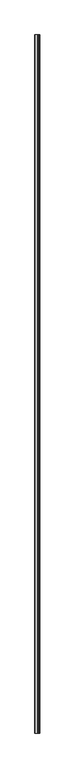
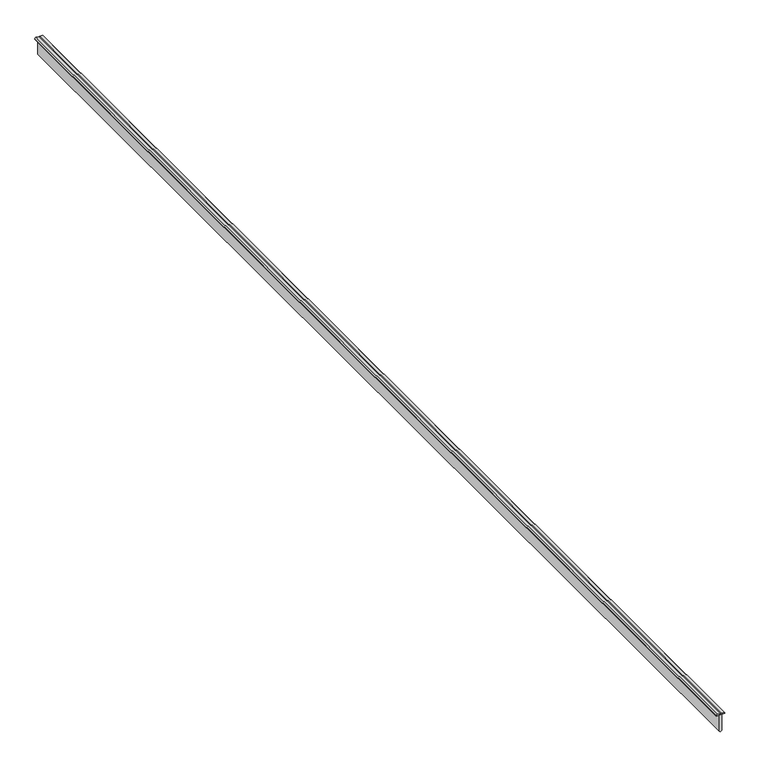
"""IFC4 building model written with IfcOpenShell, lengths in millimetres: proxy geometry, FASTENER 1:FASTENER 11861:297350 : FASTENER 1:FASTENER 11861:297350."""

from ifc_helpers import new_model, si_unit, frame, origin, place, context, project, spatial, polyline, outline, extrude, source, transform, mapped, element, save


def generic_models_a558a684(model_context):
    return source(origin(), model_context, "Body", "SweptSolid", [
        extrude(outline(polyline([(42582.1288635, 10750.5257946), (42580.5349921, 10749.2870925), (42579.6987049, 10749.2762959), (42579.6987049, 10763.5726012), (42580.508527, 10763.5726012), (42582.1023984, 10762.3338991), (42582.1023984, 10757.4548172), (42580.1167322, 10757.0482169), (42580.1167322, 10755.801112), (42581.7222633, 10755.801112), (42582.1288635, 10750.5257946)])), frame((0.0, -774.5581163, 0.0), z_axis=(0.0, 1.0, 0.0), x_axis=(0.0, 0.0, 1.0)), (0.0, 0.0, 1.0), 1999.85),
        extrude(outline(polyline([(42549.1244121, 10755.9768301), (42551.3049701, 10758.526734), (42579.6987049, 10758.526734), (42579.6987049, 10754.3198155), (42550.7399648, 10754.3198155), (42549.1244121, 10755.9768301)])), frame((0.0, -774.5581163, 0.0), z_axis=(0.0, 1.0, 0.0), x_axis=(0.0, 0.0, 1.0)), (0.0, 0.0, 1.0), 1999.85),
    ])


if __name__ == "__main__":
    model = new_model("IFC4")
    model_context = context("Model", 3, world=origin())
    ifc_project = project(units=[si_unit("LENGTHUNIT", "METRE", prefix="MILLI")], contexts=[model_context])
    site = spatial("IfcSite", under=ifc_project)
    building = spatial("IfcBuilding", under=site)
    placement = place(None, origin())
    generic_models_shape = generic_models_a558a684(model_context)
    element("IfcBuildingElementProxy", 1, Name="FASTENER 1:FASTENER 11861:297350 : FASTENER 1:FASTENER 11861:297350", ObjectType="FASTENER 1:FASTENER 11861:297350 : FASTENER 1:FASTENER 11861:297350", at=placement, inside=building, context=model_context, shape_type="MappedRepresentation", body=[
        mapped(generic_models_shape, transform((0.0, 0.0, 0.0), x_axis=(1.0, 0.0, 0.0), y_axis=(0.0, 1.0, 0.0), z_axis=(0.0, 0.0, 1.0))),
    ])
    save(model, "model.ifc")

# Revit data of these elements
# Type "FASTENER 1:FASTENER 11861:297350 : FASTENER 1:FASTENER 11861:297350"
#   NameOverride = "FASTENER 1:FASTENER 11861:297350"
#   ObjectTypeOverride = "FASTENER 1:FASTENER 11861"
#   Reference = "FASTENER 11861"
#   Category = "Generic Models"
#   Tag = "297350"
# Element 1 (IfcBuildingElementProxy, "FASTENER 1:FASTENER 11861:297350 : FASTENER 1:FASTENER 11861:297350")
#   Materials on its faces: "ENGINEERED PANCAKE HEAD FASTENER @ 12\" O.C."
# Materials
#   "ENGINEERED PANCAKE HEAD FASTENER @ 12\" O.C.": class "Unassigned", colour RGB 255 255 255, transparency 0, Cost = 0
